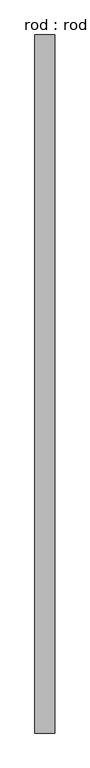
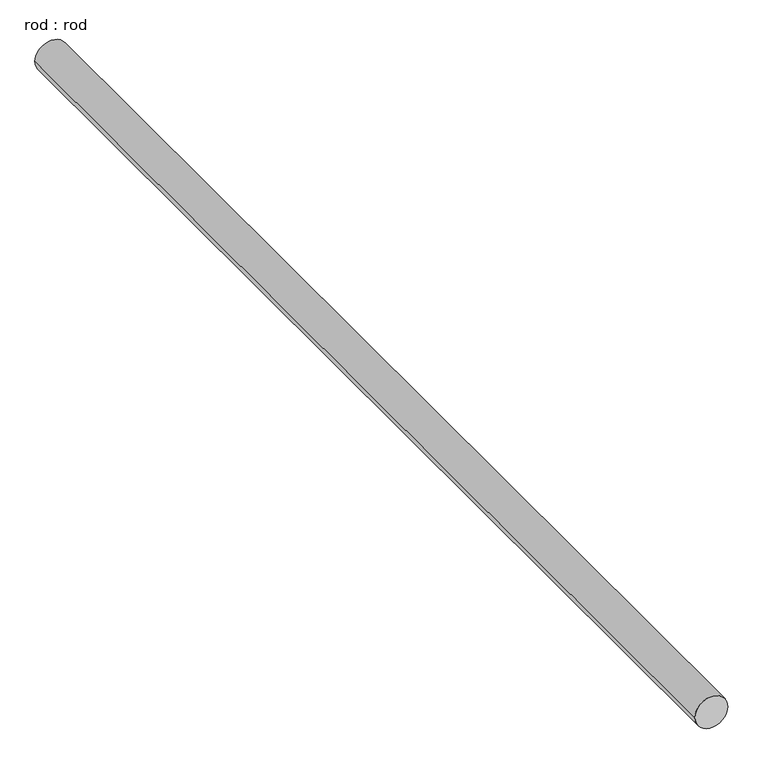
"""IFC4 building model written with IfcOpenShell, lengths in millimetres: proxy geometry, rod : rod."""

from ifc_helpers import new_model, si_unit, point, frame, frame_2d, origin, place, context, project, spatial, circle_curve, trimmed, segment, composite_curve, outline, extrude, source, transform, mapped, element, save


def rod_rod_9a81eb2d(model_context):
    return source(origin(), model_context, "Body", "SweptSolid", [
        extrude(outline(composite_curve([segment(trimmed(circle_curve(frame_2d((0.0108462, 0.0)), 200.0), [point((0.0108462, 200.0))], [point((0.0108462, -200.0))], False, "CARTESIAN"), True, "CONTINUOUS"), segment(trimmed(circle_curve(frame_2d((0.0108462, 0.0)), 200.0), [point((0.0108462, -200.0))], [point((0.0108462, 200.0))], False, "CARTESIAN"), True, "CONTINUOUS")], self_intersect=False)), frame((0.0, -2860.0585956, 0.0), z_axis=(0.0, 1.0, 0.0), x_axis=(0.0, 0.0, 1.0)), (0.0, 0.0, 1.0), 13905.5744218),
    ])


if __name__ == "__main__":
    model = new_model("IFC4")
    model_context = context("Model", 3, world=origin())
    ifc_project = project(units=[si_unit("LENGTHUNIT", "METRE", prefix="MILLI")], contexts=[model_context])
    site = spatial("IfcSite", under=ifc_project)
    building = spatial("IfcBuilding", under=site)
    placement = place(None, origin())
    rod_rod_shape = rod_rod_9a81eb2d(model_context)
    element("IfcBuildingElementProxy", 1, Name="rod : rod", ObjectType="rod : rod", at=placement, inside=building, context=model_context, shape_type="MappedRepresentation", body=[
        mapped(rod_rod_shape, transform((0.0, 0.0, 0.0), x_axis=(1.0, 0.0, 0.0), y_axis=(0.0, 1.0, 0.0), z_axis=(0.0, 0.0, 1.0))),
    ])
    save(model, "model.ifc")

# Revit data of these elements
# Type "rod : rod"
#   Default Elevation = 0
